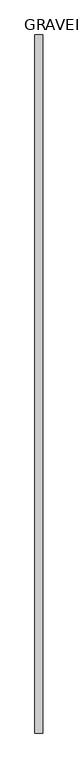
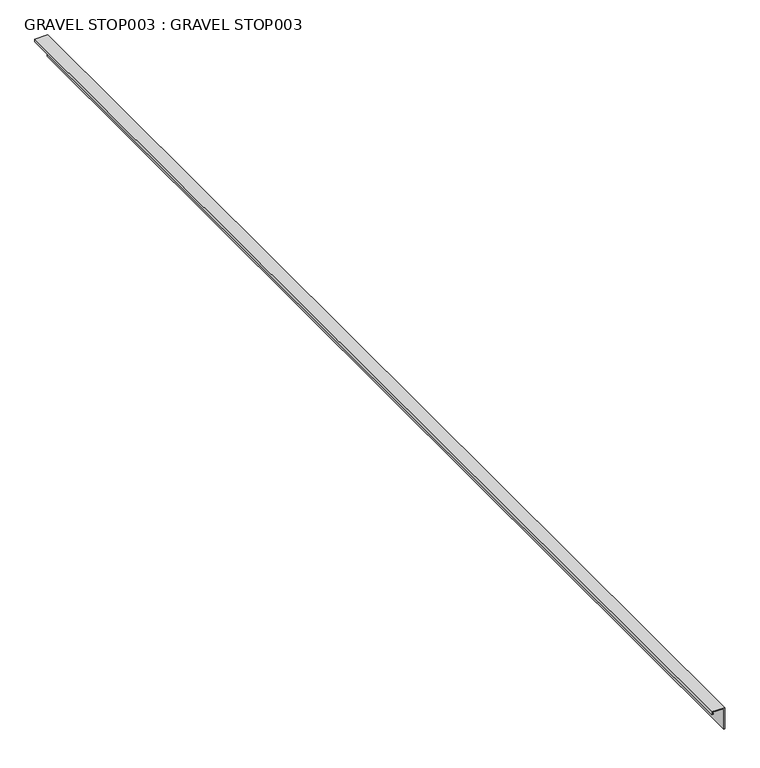
"""IFC4 building model written with IfcOpenShell, lengths in millimetres: proxy geometry, GRAVEL STOP003 : GRAVEL STOP003."""

import ifcopenshell
import ifcopenshell.guid

model = None  # the IFC model being written
_history = None  # IfcOwnerHistory: only IFC2X3 demands one
_inside = {}  # id of a spatial element -> (the spatial element, [elements in it])
_under = {}  # id of a project, library or spatial element -> (it, [spatial elements below it])
_declared = {}  # id of a project -> (the project, [libraries it declares])
_typed = {}  # id of a type object -> (the type object, [elements of that type])
_made_of = {}  # id of a material, layer set ... -> (it, [elements and type objects made of it])


def new_model(schema):
    """Start an empty IFC model of exactly this schema.

    Asked for "IFC4X3", IfcOpenShell would pick the latest addendum, in which some entities
    have other attributes; the version numbers below select the first issue.
    IFC2X3 requires an IfcOwnerHistory on every rooted entity: one is made here for all.
    """
    global model, _history
    if schema == "IFC4X3":
        model = ifcopenshell.file(schema_version=(4, 3, 0, 0))
    else:
        model = ifcopenshell.file(schema=schema)
    _inside.clear()
    _under.clear()
    _declared.clear()
    _typed.clear()
    _made_of.clear()
    _history = None
    if model.schema == "IFC2X3":
        org = make("IfcOrganization", Name="unknown")
        user = make(
            "IfcPersonAndOrganization",
            ThePerson=make("IfcPerson", FamilyName="unknown"),
            TheOrganization=org,
        )
        app = make(
            "IfcApplication",
            ApplicationDeveloper=org,
            Version="unknown",
            ApplicationFullName="unknown",
            ApplicationIdentifier="unknown",
        )
        _history = make(
            "IfcOwnerHistory",
            OwningUser=user,
            OwningApplication=app,
            ChangeAction="ADDED",
            CreationDate=0,
        )
    return model


def make(cls, **values):
    """One entity of the class cls with the attributes given. An attribute that is None is left unset."""
    return model.create_entity(
        cls, **{name: value for name, value in values.items() if value is not None}
    )


def rooted(cls, **values):
    """An entity with a GlobalId (a new one), such as an element, a storey or a relation."""
    return make(cls, GlobalId=ifcopenshell.guid.new(), OwnerHistory=_history, **values)


def si_unit(unit_type, name, prefix=None):
    """IfcSIUnit, for example si_unit("LENGTHUNIT", "METRE", prefix="MILLI")."""
    return make("IfcSIUnit", UnitType=unit_type, Prefix=prefix, Name=name)


def assignment(units):
    """IfcUnitAssignment: the units of a project."""
    return None if units is None else make("IfcUnitAssignment", Units=units)


def point(xyz):
    """IfcCartesianPoint."""
    return None if xyz is None else make("IfcCartesianPoint", Coordinates=xyz)


def direction(xyz):
    """IfcDirection."""
    return None if xyz is None else make("IfcDirection", DirectionRatios=xyz)


def frame(location, z_axis=None, x_axis=None):
    """IfcAxis2Placement3D, a coordinate frame: its origin and axes. An axis left out is left unset."""
    return make(
        "IfcAxis2Placement3D",
        Location=point(location),
        Axis=direction(z_axis),
        RefDirection=direction(x_axis),
    )


def origin():
    """The frame at (0, 0, 0) with its axes left unset."""
    return frame((0.0, 0.0, 0.0))


def place(relative_to, where):
    """IfcLocalPlacement: puts the frame where relative to a parent placement (None: the world)."""
    return make(
        "IfcLocalPlacement", PlacementRelTo=relative_to, RelativePlacement=where
    )


def context(
    kind, dimensions, precision=None, world=None, true_north=None, identifier=None
):
    """IfcGeometricRepresentationContext, for example the 3D "Model" context."""
    return make(
        "IfcGeometricRepresentationContext",
        ContextIdentifier=identifier,
        ContextType=kind,
        CoordinateSpaceDimension=dimensions,
        Precision=precision,
        WorldCoordinateSystem=world,
        TrueNorth=true_north,
    )


def project(units=None, contexts=None):
    """IfcProject with its units and contexts."""
    return rooted(
        "IfcProject",
        Name="project",
        RepresentationContexts=contexts,
        UnitsInContext=assignment(units),
    )


def spatial(cls, under=None, at=None, **own):
    """A site, building, storey or space (cls), placed at a placement, below another one or the project."""
    s = rooted(cls, ObjectPlacement=at, **own)
    if under is not None:
        _under.setdefault(under.id(), (under, []))[1].append(s)
    return s


def polyline(points):
    """IfcPolyline through the points."""
    return make("IfcPolyline", Points=[point(p) for p in points])


def outline(outer, holes=None, kind="AREA"):
    """IfcArbitraryClosedProfileDef: a profile drawn as a closed curve; with holes, ...WithVoids."""
    if holes is None:
        return make("IfcArbitraryClosedProfileDef", ProfileType=kind, OuterCurve=outer)
    return make(
        "IfcArbitraryProfileDefWithVoids",
        ProfileType=kind,
        OuterCurve=outer,
        InnerCurves=holes,
    )


def extrude(swept, where, along, depth):
    """IfcExtrudedAreaSolid: the profile swept, set in the frame where, extruded along a direction by depth."""
    return make(
        "IfcExtrudedAreaSolid",
        SweptArea=swept,
        Position=where,
        ExtrudedDirection=direction(along),
        Depth=depth,
    )


def shape(context_of_items, identifier, shape_type, items):
    """IfcShapeRepresentation: the items that make up one representation, for example the "Body"."""
    return make(
        "IfcShapeRepresentation",
        ContextOfItems=context_of_items,
        RepresentationIdentifier=identifier,
        RepresentationType=shape_type,
        Items=items,
    )


def source(mapping_origin, context_of_items, identifier, shape_type, items):
    """IfcRepresentationMap: a shape defined once, which mapped items show again and again."""
    return make(
        "IfcRepresentationMap",
        MappingOrigin=mapping_origin,
        MappedRepresentation=shape(context_of_items, identifier, shape_type, items),
    )


def transform(
    local_origin,
    x_axis=None,
    y_axis=None,
    z_axis=None,
    scale=None,
    scale2=None,
    scale3=None,
    uniform=True,
):
    """IfcCartesianTransformationOperator3D, or its non-uniform kind. x_axis, y_axis, z_axis: its Axis1, 2, 3."""
    if uniform:
        return make(
            "IfcCartesianTransformationOperator3D",
            Axis1=direction(x_axis),
            Axis2=direction(y_axis),
            LocalOrigin=point(local_origin),
            Scale=scale,
            Axis3=direction(z_axis),
        )
    return make(
        "IfcCartesianTransformationOperator3DnonUniform",
        Axis1=direction(x_axis),
        Axis2=direction(y_axis),
        LocalOrigin=point(local_origin),
        Scale=scale,
        Axis3=direction(z_axis),
        Scale2=scale2,
        Scale3=scale3,
    )


def mapped(mapping_source, mapping_target):
    """IfcMappedItem: shows the shape of a source again, moved by a transform."""
    return make(
        "IfcMappedItem", MappingSource=mapping_source, MappingTarget=mapping_target
    )


def made_of(thing, what):
    """Note that an element or type object is made of a material, layer set ...; save() writes the relation."""
    if what is not None:
        _made_of.setdefault(what.id(), (what, []))[1].append(thing)
    return thing


def element(
    cls,
    number,
    at=None,
    inside=None,
    cuts=None,
    type_object=None,
    material=None,
    context=None,
    identifier="Body",
    shape_type=None,
    held_by="IfcProductDefinitionShape",
    body=None,
    shapes=None,
    **own,
):
    """One element of the class cls, such as IfcWall. Its Tag is "e" and its number.

    at: its placement. inside: the storey or other place that contains it. cuts: it is an
    opening in that element (IfcRelVoidsElement). A single representation is given by context,
    identifier, shape_type and body (its items); several are given by shapes. held_by: the class
    of the entity that holds the representations. save() writes the other relations.
    """
    e = rooted(cls, Tag="e%d" % number, ObjectPlacement=at, **own)
    if body is not None:
        shapes = [shape(context, identifier, shape_type, body)]
    if shapes is not None:
        e.Representation = make(held_by, Representations=shapes)
    if inside is not None:
        _inside.setdefault(inside.id(), (inside, []))[1].append(e)
    if cuts is not None:
        rooted(
            "IfcRelVoidsElement", RelatingBuildingElement=cuts, RelatedOpeningElement=e
        )
    if type_object is not None:
        _typed.setdefault(type_object.id(), (type_object, []))[1].append(e)
    return made_of(e, material)


def aggregate(whole, parts):
    """IfcRelAggregates: a whole, such as a stair, and the parts it consists of."""
    return rooted("IfcRelAggregates", RelatingObject=whole, RelatedObjects=parts)


def save(model, path):
    """Write the relations noted so far, then the file.

    IfcRelAggregates (storeys below a building ...), IfcRelContainedInSpatialStructure (elements
    in a storey), IfcRelDefinesByType, IfcRelAssociatesMaterial and IfcRelDeclares: one each for
    every whole, place, type object, material and project.
    """
    for whole, parts in _under.values():
        aggregate(whole, parts)
    for where, things in _inside.values():
        rooted(
            "IfcRelContainedInSpatialStructure",
            RelatedElements=things,
            RelatingStructure=where,
        )
    for kind, things in _typed.values():
        rooted("IfcRelDefinesByType", RelatedObjects=things, RelatingType=kind)
    for what, things in _made_of.values():
        rooted("IfcRelAssociatesMaterial", RelatedObjects=things, RelatingMaterial=what)
    for by, libraries in _declared.values():
        rooted("IfcRelDeclares", RelatingContext=by, RelatedDefinitions=libraries)
    model.write(path)


def gravel_stop003_gravel_stop003_12768274(model_context):
    return source(origin(), model_context, "Body", "SweptSolid", [
        extrude(outline(polyline([(40234.4061757, -5021.258828), (40197.5761757, -5021.258828), (40197.5761757, -5019.988828), (40235.6761757, -5019.988828), (40235.6761757, -5042.213828), (40230.9263757, -5042.213828), (40230.9263757, -5039.2113716), (40232.1963757, -5039.2113716), (40232.1963757, -5040.943828), (40234.4061757, -5040.943828), (40234.4061757, -5021.258828)])), frame((0.0, -1052.8906573, 0.0), z_axis=(0.0, 1.0, 0.0), x_axis=(0.0, 0.0, 1.0)), (0.0, 0.0, 1.0), 2000.25),
    ])


if __name__ == "__main__":
    model = new_model("IFC4")
    model_context = context("Model", 3, world=origin())
    ifc_project = project(units=[si_unit("LENGTHUNIT", "METRE", prefix="MILLI")], contexts=[model_context])
    site = spatial("IfcSite", under=ifc_project)
    building = spatial("IfcBuilding", under=site)
    placement = place(None, origin())
    gravel_stop003_gravel_stop003_shape = gravel_stop003_gravel_stop003_12768274(model_context)
    element("IfcBuildingElementProxy", 1, Name="GRAVEL STOP003 : GRAVEL STOP003", ObjectType="GRAVEL STOP003 : GRAVEL STOP003", at=placement, inside=building, context=model_context, shape_type="MappedRepresentation", body=[
        mapped(gravel_stop003_gravel_stop003_shape, transform((0.0, 0.0, 0.0), x_axis=(1.0, 0.0, 0.0), y_axis=(0.0, 1.0, 0.0), z_axis=(0.0, 0.0, 1.0))),
    ])
    save(model, "model.ifc")

# Revit data of these elements
# Type "GRAVEL STOP003 : GRAVEL STOP003"
#   NameOverride = "GRAVEL STOP003"
# Element 1 (IfcBuildingElementProxy, "GRAVEL STOP003 : GRAVEL STOP003")
#   Materials on its faces: "COPPER STUCCO J BEAD"
# Materials
#   "COPPER STUCCO J BEAD": class "Unassigned", colour RGB 251 232 155, transparency 0, Cost = 0
